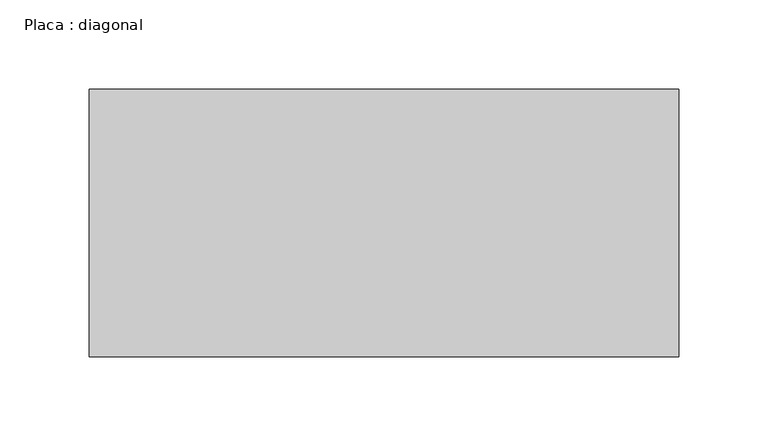
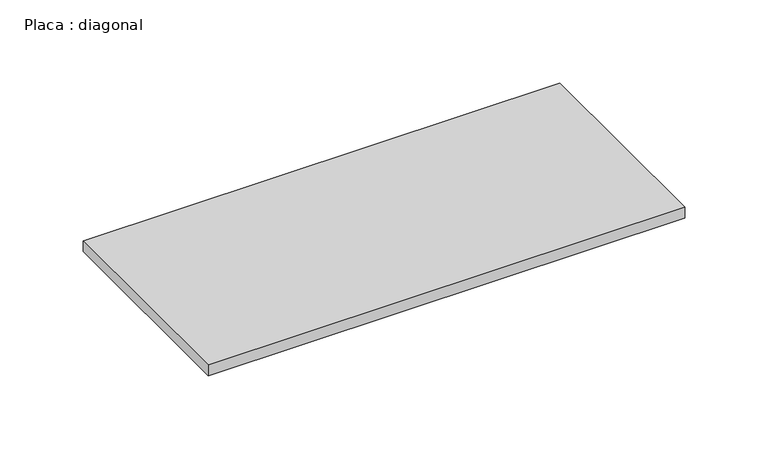
"""IFC4 building model written with IfcOpenShell, lengths in millimetres: beam geometry, Placa : diagonal."""

from ifc_helpers import new_model, si_unit, frame, origin, place, context, project, spatial, polyline, outline, extrude, source, transform, mapped, element, save


def placa_diagonal_c0f04519(model_context):
    return source(origin(), model_context, "Body", "SweptSolid", [
        extrude(outline(polyline([(165.1705218, 75.0), (165.1705218, -75.0), (-165.4962732, -75.0), (-165.4962732, 75.0), (165.1705218, 75.0)])), frame((0.0, 0.0, -4.0), z_axis=(0.0, 0.0, 1.0), x_axis=(1.0, 0.0, 0.0)), (0.0, 0.0, 1.0), 8.0),
    ])


if __name__ == "__main__":
    model = new_model("IFC4")
    model_context = context("Model", 3, world=origin())
    ifc_project = project(units=[si_unit("LENGTHUNIT", "METRE", prefix="MILLI")], contexts=[model_context])
    site = spatial("IfcSite", under=ifc_project)
    building = spatial("IfcBuilding", under=site)
    placement = place(None, origin())
    placa_diagonal_shape = placa_diagonal_c0f04519(model_context)
    element("IfcBeam", 1, ObjectType="Placa : diagonal", at=placement, inside=building, context=model_context, shape_type="MappedRepresentation", body=[
        mapped(placa_diagonal_shape, transform((0.0, 0.0, 0.0), x_axis=(1.0, 0.0, 0.0), y_axis=(0.0, 1.0, 0.0), z_axis=(0.0, 0.0, 1.0))),
    ])
    save(model, "model.ifc")

# Revit data of these elements
# Type "Placa : diagonal"
#   W = 0
#   Length [instance default] = 1.50 m
#   b = 0.15 m
#   d = 0.008 m
#   A = 0 m²
#   Structural Material [instance default] = Aço, 45-345
# Element 1 (IfcBeam, "Placa : diagonal")
#   Materials on its faces: "Aço, 45-345"
# Materials
#   "Aço, 45-345": class "Metal", colour RGB 247 247 247, transparency 0, Description = "Aço 345 MPa", Cost = 0
